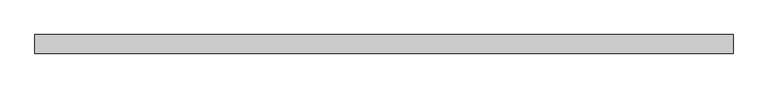
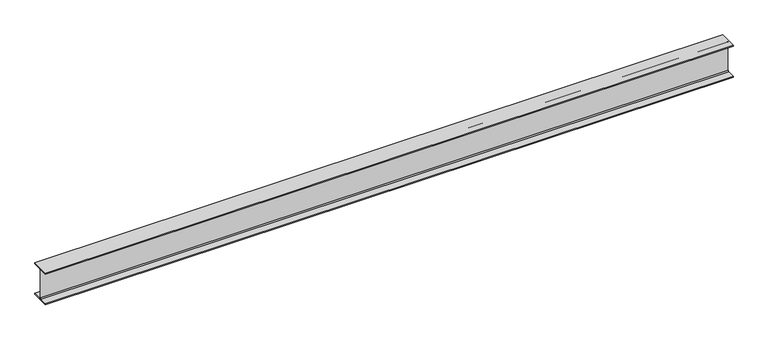
"""IFC4 building model written with IfcOpenShell, lengths in millimetres: beam geometry, Old_Steel Beam_H-KSD3502 : H_SB_ASB_H-400×200x8x13."""

from ifc_helpers import new_model, si_unit, point, frame, frame_2d, origin, place, context, project, spatial, polyline, circle_curve, trimmed, segment, composite_curve, outline, extrude, source, transform, mapped, element, save


def beam_a60eb2c5(model_context):
    return source(origin(), model_context, "Body", "SweptSolid", [
        extrude(outline(composite_curve([segment(polyline([(82.5, -141.5), (82.5, -151.7), (-82.5, -151.7), (-82.5, -141.5), (-11.9, -141.5)]), True, "CONTINUOUS"), segment(trimmed(circle_curve(frame_2d((-11.9, -132.6)), 8.9), [point((-11.9, -141.5))], [point((-3.0, -132.6))], True, "CARTESIAN"), True, "CONTINUOUS"), segment(polyline([(-3.0, -132.6), (-3.0, 132.6)]), True, "CONTINUOUS"), segment(trimmed(circle_curve(frame_2d((-11.9, 132.6)), 8.9), [point((-3.0, 132.6))], [point((-11.9, 141.5))], True, "CARTESIAN"), True, "CONTINUOUS"), segment(polyline([(-11.9, 141.5), (-82.5, 141.5), (-82.5, 151.7), (82.5, 151.7), (82.5, 141.5), (11.9, 141.5)]), True, "CONTINUOUS"), segment(trimmed(circle_curve(frame_2d((11.9, 132.6)), 8.9), [point((11.9, 141.5))], [point((3.0, 132.6))], True, "CARTESIAN"), True, "CONTINUOUS"), segment(polyline([(3.0, 132.6), (3.0, -132.6)]), True, "CONTINUOUS"), segment(trimmed(circle_curve(frame_2d((11.9, -132.6)), 8.9), [point((3.0, -132.6))], [point((11.9, -141.5))], True, "CARTESIAN"), True, "CONTINUOUS"), segment(polyline([(11.9, -141.5), (82.5, -141.5)]), True, "CONTINUOUS")], self_intersect=False)), frame((-3154.8, 0.0, 0.0), z_axis=(1.0, 0.0, 0.0), x_axis=(0.0, 1.0, 0.0)), (0.0, 0.0, 1.0), 6192.1),
    ])


if __name__ == "__main__":
    model = new_model("IFC4")
    model_context = context("Model", 3, world=origin())
    ifc_project = project(units=[si_unit("LENGTHUNIT", "METRE", prefix="MILLI")], contexts=[model_context])
    site = spatial("IfcSite", under=ifc_project)
    building = spatial("IfcBuilding", under=site)
    placement = place(None, origin())
    beam_shape = beam_a60eb2c5(model_context)
    element("IfcBeam", 1, ObjectType="Old_Steel Beam_H-KSD3502 : H_SB_ASB_H-400×200x8x13", at=placement, inside=building, context=model_context, shape_type="MappedRepresentation", body=[
        mapped(beam_shape, transform((0.0, 0.0, 0.0), x_axis=(1.0, 0.0, 0.0), y_axis=(0.0, 1.0, 0.0), z_axis=(0.0, 0.0, 1.0))),
    ])
    save(model, "model.ifc")

# Revit data of these elements
# Type "Old_Steel Beam_H-KSD3502 : H_SB_ASB_H-400×200x8x13"
#   Width = 20.0 cm
#   Web Thickness = 0.8 cm
#   Web Fillet = 1.6 cm
#   Warping Constant = 648999.0 cm⁶
#   Torsional Moment of Inertia = 35.8981 cm⁴
#   Torsional Modulus = 1.0 cm³
#   Section Area = 84.12 cm²
#   Plastic Modulus weak axis = 268.0 cm³
#   Plastic Modulus strong axis = 1330.0 cm³
#   Perimeter = 1.56 m²/m
#   Nominal Weight = 66.00 kgf/m
#   Moment of Inertia weak axis = 1740.00 cm⁴
#   Moment of Inertia strong axis = 23700.00 cm⁴
#   Height = 40.0 cm
#   Flange Thickness = 1.3 cm
#   Elastic Modulus weak axis = 174.0 cm³
#   Elastic Modulus strong axis = 1190.0 cm³
#   Centroid Vertical = 20.0 cm
#   Centroid Horizontal = 10.0 cm
#   Length [instance default] = 1.5240 m
#   Structural Material [instance default] = Steel, 45-345
#   Assembly Code = ""
# Element 1 (IfcBeam, "Old_Steel Beam_H-KSD3502 : H_SB_ASB_H-400×200x8x13")
#   Structural Material = none
# Materials
#   "Steel, 45-345": class "Metal", colour RGB 189 187 185, transparency 0, Description = "Steel 345 MPa", Cost = 0
